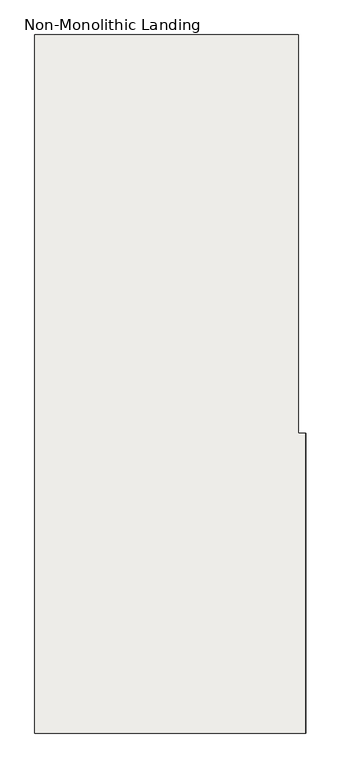
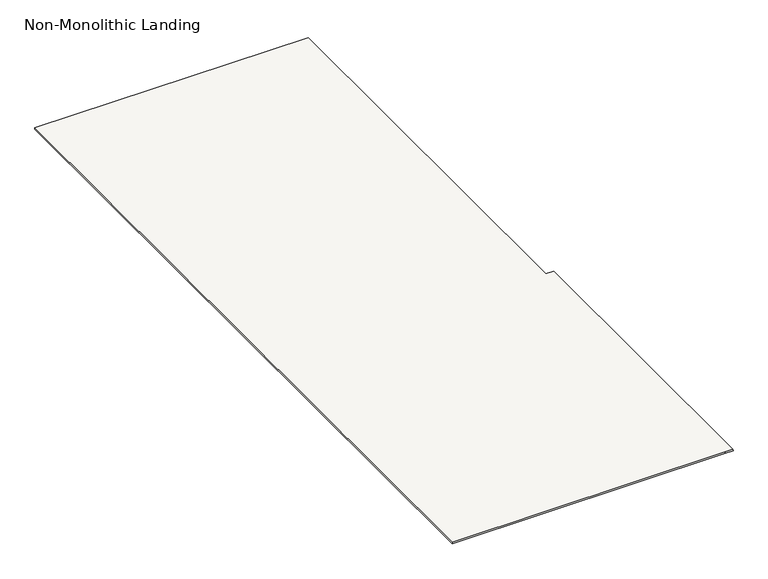
"""IFC4 building model written with IfcOpenShell, lengths in millimetres: slab geometry, Non-Monolithic Landing."""

from ifc_helpers import new_model, si_unit, origin, place, context, project, spatial, faceted_brep, source, transform, mapped, element, save


def non_monolithic_landing_46507575(model_context):
    return source(origin(), model_context, "Body", "Brep", [
        faceted_brep([(13356.0590357, 10220.4345331, 4088.8888889), (13356.9027857, 10220.4345331, 4082.8888889), (13356.9027857, 11470.4345331, 4082.8888889), (13356.0590357, 11470.4345331, 4088.8888889), (13325.0, 13130.4345331, 4088.8888889), (12225.0, 13130.4345331, 4088.8888889), (12225.0, 10220.4345331, 4088.8888889), (13325.0, 10220.4345331, 4088.8888889), (13325.0, 11470.4345331, 4088.8888889), (13325.0, 12030.4345331, 4088.8888889), (12225.0, 10220.4345331, 4082.8888889), (12225.0, 13130.4345331, 4082.8888889), (13324.15625, 13130.4345331, 4082.8888889), (13324.15625, 12030.4345331, 4082.8888889), (13325.0, 12030.4345331, 4082.8888889), (13325.0, 11470.4345331, 4082.8888889), (13325.0, 10220.4345331, 4082.8888889)], [[[0, 1, 2, 3]], [[4, 5, 6, 7, 0, 3, 8, 9]], [[10, 11, 12, 13, 14, 15, 2, 1, 16]], [[9, 8, 15, 14]], [[0, 7, 16, 1]], [[7, 6, 10, 16]], [[6, 5, 11, 10]], [[5, 4, 12, 11]], [[13, 9, 14]], [[9, 13, 12, 4]], [[8, 3, 2, 15]]]),
    ])


if __name__ == "__main__":
    model = new_model("IFC4")
    model_context = context("Model", 3, world=origin())
    ifc_project = project(units=[si_unit("LENGTHUNIT", "METRE", prefix="MILLI")], contexts=[model_context])
    site = spatial("IfcSite", under=ifc_project)
    building = spatial("IfcBuilding", under=site)
    placement = place(None, origin())
    non_monolithic_landing_shape = non_monolithic_landing_46507575(model_context)
    element("IfcSlab", 1, ObjectType="Non-Monolithic Landing", at=placement, inside=building, context=model_context, shape_type="MappedRepresentation", body=[
        mapped(non_monolithic_landing_shape, transform((0.0, 0.0, 0.0), x_axis=(1.0, 0.0, 0.0), y_axis=(0.0, 1.0, 0.0), z_axis=(0.0, 0.0, 1.0))),
    ])
    save(model, "model.ifc")

# Revit data of these elements
# Element 1 (IfcSlab, "Non-Monolithic Landing")
#   Materials on its faces: "Steel, Paint Finish, Dark Gray"
# Materials
#   "Steel, Paint Finish, Dark Gray": class "Metal", colour RGB 89 89 89, transparency 0, Description = "Steel, paint finish, dark gray, glossy", Cost = 0
